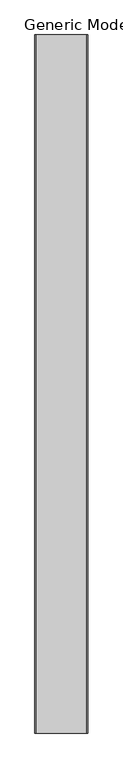
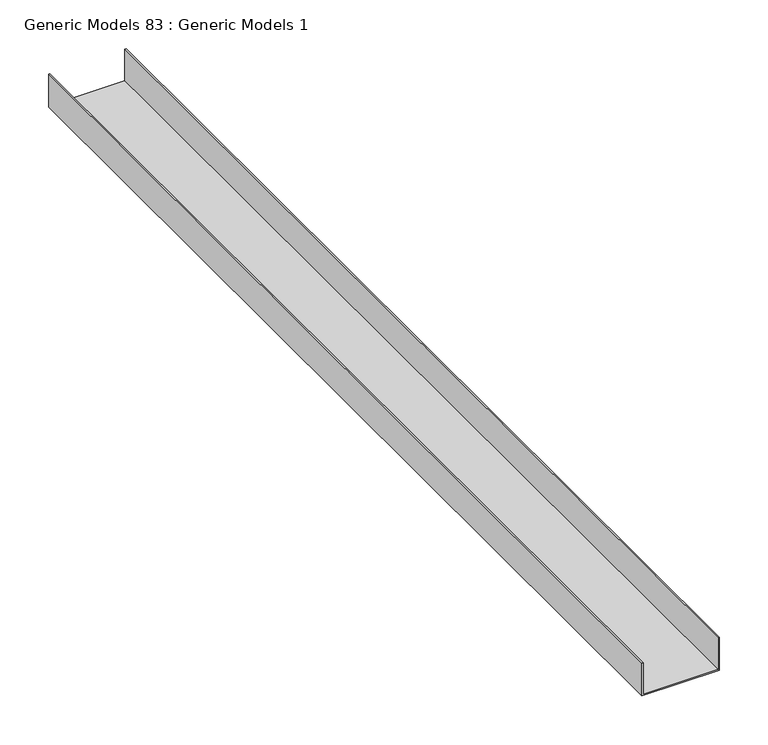
"""IFC4 building model written with IfcOpenShell, lengths in millimetres: proxy geometry, Generic Models 83 : Generic Models 1."""

from ifc_helpers import new_model, si_unit, frame, origin, place, context, project, spatial, polyline, outline, extrude, source, transform, mapped, element, save


def generic_models_83_generic_models_1_169b68fe(model_context):
    return source(origin(), model_context, "Body", "SweptSolid", [
        extrude(outline(polyline([(2067.2531297, 46935.8735531), (2108.5281297, 46935.8735531), (2108.5281297, 46934.2860531), (2068.8406297, 46934.2860531), (2068.8406297, 46845.3860531), (2108.5281297, 46845.3860531), (2108.5281297, 46843.7985531), (2067.2531297, 46843.7985531), (2067.2531297, 46935.8735531)])), frame((0.0, 0.0, 0.0), z_axis=(0.0, 1.0, 0.0), x_axis=(0.0, 0.0, 1.0)), (0.0, 0.0, 1.0), 1219.2),
    ])


if __name__ == "__main__":
    model = new_model("IFC4")
    model_context = context("Model", 3, world=origin())
    ifc_project = project(units=[si_unit("LENGTHUNIT", "METRE", prefix="MILLI")], contexts=[model_context])
    site = spatial("IfcSite", under=ifc_project)
    building = spatial("IfcBuilding", under=site)
    placement = place(None, origin())
    generic_models_83_generic_models_1_shape = generic_models_83_generic_models_1_169b68fe(model_context)
    element("IfcBuildingElementProxy", 1, Name="Generic Models 83 : Generic Models 1", ObjectType="Generic Models 83 : Generic Models 1", at=placement, inside=building, context=model_context, shape_type="MappedRepresentation", body=[
        mapped(generic_models_83_generic_models_1_shape, transform((0.0, 0.0, 0.0), x_axis=(1.0, 0.0, 0.0), y_axis=(0.0, 1.0, 0.0), z_axis=(0.0, 0.0, 1.0))),
    ])
    save(model, "model.ifc")

# Revit data of these elements
# Element 1 (IfcBuildingElementProxy, "Generic Models 83 : Generic Models 1")
#   Materials on its faces: "DEEP LEG OF DEFLECTION TRACK (2\" MIN. DEFLECTION)"
# Materials
#   "DEEP LEG OF DEFLECTION TRACK (2\" MIN. DEFLECTION)": class "Unassigned", colour RGB 210 209 208, transparency 0, Keynote = "M05121300.02", Cost = 0
